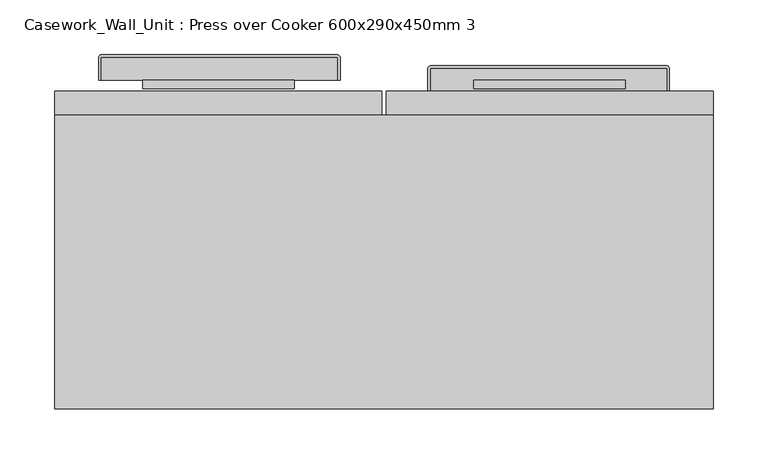
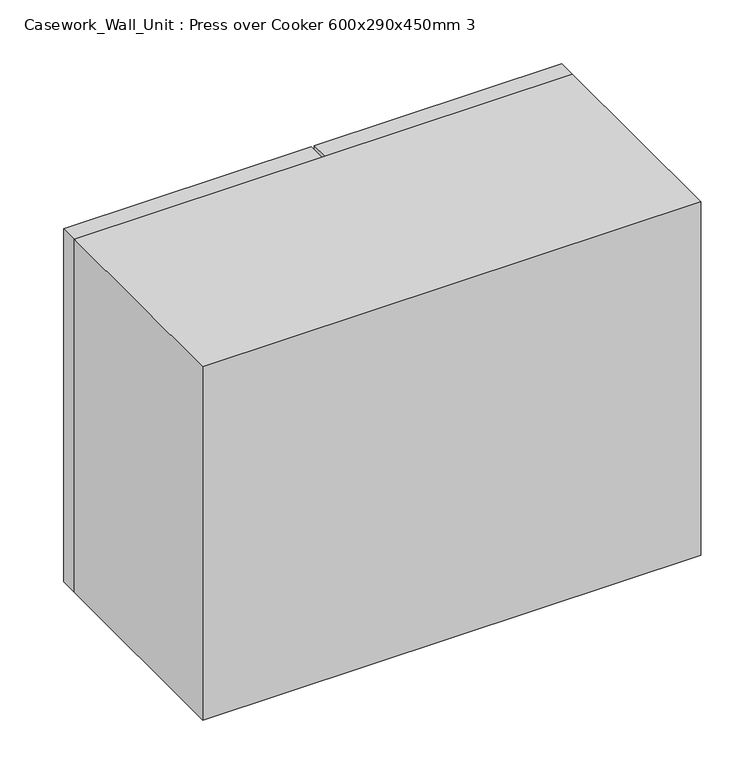
"""IFC4 building model written with IfcOpenShell, lengths in millimetres: furniture geometry, Casework_Wall_Unit : Press over Cooker 600x290x450mm 3."""

from ifc_helpers import new_model, si_unit, point, frame, frame_2d, origin, place, context, project, spatial, polyline, circle_curve, trimmed, segment, composite_curve, outline, extrude, faceted_brep, source, transform, mapped, element, save


def casework_wall_unit_press_over_cooker_600x290x450mm_3_e573720d(model_context):
    return source(origin(), model_context, "Body", "SolidModel", [
        extrude(outline(composite_curve([segment(polyline([(-83.0, 365.0), (-83.0, 385.5)]), True, "CONTINUOUS"), segment(trimmed(circle_curve(frame_2d((-82.5, 385.5)), 0.5), [point((-83.0, 385.5))], [point((-82.5, 386.0))], False, "CARTESIAN"), True, "CONTINUOUS"), segment(polyline([(-82.5, 386.0), (132.5, 386.0)]), True, "CONTINUOUS"), segment(trimmed(circle_curve(frame_2d((132.5, 385.5)), 0.5), [point((132.5, 386.0))], [point((133.0, 385.5))], False, "CARTESIAN"), True, "CONTINUOUS"), segment(polyline([(133.0, 385.5), (133.0, 365.0), (-83.0, 365.0)]), True, "CONTINUOUS")], self_intersect=False)), frame((0.0, 0.0, 1639.5509264), z_axis=(0.0, 0.0, 1.0), x_axis=(1.0, 0.0, 0.0)), (0.0, 0.0, 1.0), 6.4890959),
        extrude(outline(composite_curve([segment(polyline([(-85.0, 365.0), (-85.0, 385.5)]), True, "CONTINUOUS"), segment(trimmed(circle_curve(frame_2d((-82.5, 385.5)), 2.5), [point((-85.0, 385.5))], [point((-82.5, 388.0))], False, "CARTESIAN"), True, "CONTINUOUS"), segment(polyline([(-82.5, 388.0), (132.5, 388.0)]), True, "CONTINUOUS"), segment(trimmed(circle_curve(frame_2d((132.5, 385.5)), 2.5), [point((132.5, 388.0))], [point((135.0, 385.5))], False, "CARTESIAN"), True, "CONTINUOUS"), segment(polyline([(135.0, 385.5), (135.0, 365.0), (133.0, 365.0), (133.0, 385.5)]), True, "CONTINUOUS"), segment(trimmed(circle_curve(frame_2d((132.5, 385.5)), 0.5), [point((133.0, 385.5))], [point((132.5, 386.0))], True, "CARTESIAN"), True, "CONTINUOUS"), segment(polyline([(132.5, 386.0), (-82.5, 386.0)]), True, "CONTINUOUS"), segment(trimmed(circle_curve(frame_2d((-82.5, 385.5)), 0.5), [point((-82.5, 386.0))], [point((-83.0, 385.5))], True, "CARTESIAN"), True, "CONTINUOUS"), segment(polyline([(-83.0, 385.5), (-83.0, 365.0), (-85.0, 365.0)]), True, "CONTINUOUS")], self_intersect=False)), frame((0.0, 0.0, 1636.7855373), z_axis=(0.0, 0.0, 1.0), x_axis=(1.0, 0.0, 0.0)), (0.0, 0.0, 1.0), 12.0),
        extrude(outline(composite_curve([segment(polyline([(217.0, 355.0), (217.0, 375.5)]), True, "CONTINUOUS"), segment(trimmed(circle_curve(frame_2d((217.5, 375.5)), 0.5), [point((217.0, 375.5))], [point((217.5, 376.0))], False, "CARTESIAN"), True, "CONTINUOUS"), segment(polyline([(217.5, 376.0), (432.5, 376.0)]), True, "CONTINUOUS"), segment(trimmed(circle_curve(frame_2d((432.5, 375.5)), 0.5), [point((432.5, 376.0))], [point((433.0, 375.5))], False, "CARTESIAN"), True, "CONTINUOUS"), segment(polyline([(433.0, 375.5), (433.0, 355.0), (217.0, 355.0)]), True, "CONTINUOUS")], self_intersect=False)), frame((0.0, 0.0, 1639.5509264), z_axis=(0.0, 0.0, 1.0), x_axis=(1.0, 0.0, 0.0)), (0.0, 0.0, 1.0), 6.4890959),
        extrude(outline(composite_curve([segment(polyline([(215.0, 355.0), (215.0, 375.5)]), True, "CONTINUOUS"), segment(trimmed(circle_curve(frame_2d((217.5, 375.5)), 2.5), [point((215.0, 375.5))], [point((217.5, 378.0))], False, "CARTESIAN"), True, "CONTINUOUS"), segment(polyline([(217.5, 378.0), (432.5, 378.0)]), True, "CONTINUOUS"), segment(trimmed(circle_curve(frame_2d((432.5, 375.5)), 2.5), [point((432.5, 378.0))], [point((435.0, 375.5))], False, "CARTESIAN"), True, "CONTINUOUS"), segment(polyline([(435.0, 375.5), (435.0, 355.0), (433.0, 355.0), (433.0, 375.5)]), True, "CONTINUOUS"), segment(trimmed(circle_curve(frame_2d((432.5, 375.5)), 0.5), [point((433.0, 375.5))], [point((432.5, 376.0))], True, "CARTESIAN"), True, "CONTINUOUS"), segment(polyline([(432.5, 376.0), (217.5, 376.0)]), True, "CONTINUOUS"), segment(trimmed(circle_curve(frame_2d((217.5, 375.5)), 0.5), [point((217.5, 376.0))], [point((217.0, 375.5))], True, "CARTESIAN"), True, "CONTINUOUS"), segment(polyline([(217.0, 375.5), (217.0, 355.0), (215.0, 355.0)]), True, "CONTINUOUS")], self_intersect=False)), frame((0.0, 0.0, 1636.7855373), z_axis=(0.0, 0.0, 1.0), x_axis=(1.0, 0.0, 0.0)), (0.0, 0.0, 1.0), 12.0),
        extrude(outline(polyline([(395.0, 357.0), (257.0, 357.0), (257.0, 365.0), (395.0, 365.0), (395.0, 357.0)])), frame((0.0, 0.0, 1689.7855373), z_axis=(0.0, 0.0, 1.0), x_axis=(1.0, 0.0, 0.0)), (0.0, 0.0, 1.0), 270.0),
        extrude(outline(polyline([(93.0, 357.0), (-45.0, 357.0), (-45.0, 365.0), (93.0, 365.0), (93.0, 357.0)])), frame((0.0, 0.0, 1689.7855373), z_axis=(0.0, 0.0, 1.0), x_axis=(1.0, 0.0, 0.0)), (0.0, 0.0, 1.0), 270.0),
        faceted_brep([(453.0, 333.0, 1611.7855373), (-103.0, 333.0, 1611.7855373), (-103.0, 87.0, 1611.7855373), (453.0, 87.0, 1611.7855373), (475.0, 333.0, 1589.7855373), (475.0, 65.0, 1589.7855373), (-125.0, 65.0, 1589.7855373), (-125.0, 333.0, 1589.7855373), (-125.0, 333.0, 2039.7855373), (475.0, 333.0, 2039.7855373), (453.0, 333.0, 2017.7855373), (-103.0, 333.0, 2017.7855373), (-125.0, 65.0, 2039.7855373), (475.0, 65.0, 2039.7855373), (453.0, 87.0, 2017.7855373), (-103.0, 87.0, 2017.7855373)], [[[0, 1, 2, 3]], [[4, 5, 6, 7]], [[8, 9, 4, 7], [0, 10, 11, 1]], [[8, 7, 6, 12]], [[12, 6, 5, 13]], [[13, 5, 4, 9]], [[10, 0, 3, 14]], [[14, 3, 2, 15]], [[1, 11, 15, 2]], [[9, 8, 12, 13]], [[11, 10, 14, 15]]]),
        extrude(outline(polyline([(2039.7855373, 177.0), (1589.7855373, 177.0), (1589.7855373, 475.0), (2039.7855373, 475.0), (2039.7855373, 177.0)]), holes=[polyline([(1959.7855373, 257.0), (1959.7855373, 395.0), (1689.7855373, 395.0), (1689.7855373, 257.0), (1959.7855373, 257.0)])]), frame((0.0, 333.0, 0.0), z_axis=(0.0, 1.0, 0.0), x_axis=(0.0, 0.0, 1.0)), (0.0, 0.0, 1.0), 22.0),
        extrude(outline(polyline([(2039.7855373, 173.0), (2039.7855373, -125.0), (1589.7855373, -125.0), (1589.7855373, 173.0), (2039.7855373, 173.0)]), holes=[polyline([(1959.7855373, 93.0), (1689.7855373, 93.0), (1689.7855373, -45.0), (1959.7855373, -45.0), (1959.7855373, 93.0)])]), frame((0.0, 333.0, 0.0), z_axis=(0.0, 1.0, 0.0), x_axis=(0.0, 0.0, 1.0)), (0.0, 0.0, 1.0), 22.0),
    ])


if __name__ == "__main__":
    model = new_model("IFC4")
    model_context = context("Model", 3, world=origin())
    ifc_project = project(units=[si_unit("LENGTHUNIT", "METRE", prefix="MILLI")], contexts=[model_context])
    site = spatial("IfcSite", under=ifc_project)
    building = spatial("IfcBuilding", under=site)
    placement = place(None, origin())
    casework_wall_unit_press_over_cooker_600x290x450mm_3_shape = casework_wall_unit_press_over_cooker_600x290x450mm_3_e573720d(model_context)
    element("IfcFurniture", 1, ObjectType="Casework_Wall_Unit : Press over Cooker 600x290x450mm 3", at=placement, inside=building, context=model_context, shape_type="MappedRepresentation", body=[
        mapped(casework_wall_unit_press_over_cooker_600x290x450mm_3_shape, transform((0.0, 0.0, 0.0), x_axis=(1.0, 0.0, 0.0), y_axis=(0.0, 1.0, 0.0), z_axis=(0.0, 0.0, 1.0))),
    ])
    save(model, "model.ifc")

# Revit data of these elements
# Type "Casework_Wall_Unit : Press over Cooker 600x290x450mm 3"
#   Manufacturer = "Revit"
#   Keynote = "N10"
#   Assembly Code = "C1030400"
#   Width = 600 mm
#   Height = 450 mm
#   Depth = 290 mm
#   Material Panel = Cabinets - Panel/Glass
#   Material Handle = Cabinets - Handles
#   Material Cabinet = Cabinets
# Element 1 (IfcFurniture, "Casework_Wall_Unit : Press over Cooker 600x290x450mm 3")
#   Materials on its faces: "Cabinets - Handles", "Cabinets", "Cabinets - Panel/Glass"
# Materials
#   "Cabinets - Panel/Glass": class "Miscellaneous", colour RGB 252 255 255, transparency 0.72
#   "Cabinets - Handles": class "Metal", colour RGB 57 57 57, transparency 0
#   "Cabinets": class "Miscellaneous", colour RGB 249 249 249, transparency 0
